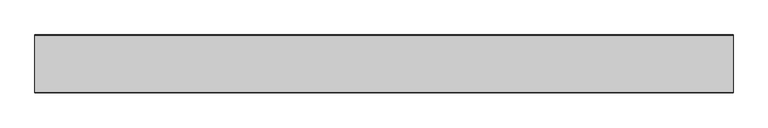
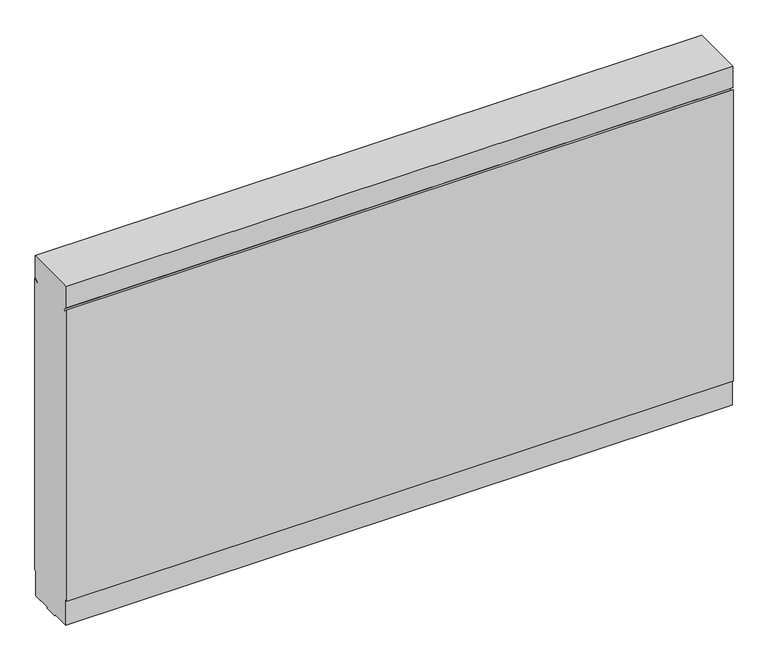
"""IFC4 building model written with IfcOpenShell, lengths in millimetres: proxy geometry, Generic Models 7:Generic Models 1:5:Generic Models 1:5 : Generic Models 7:Generic Models 1:337419:18 : Generic Models 7:Generic Models 1:5:Generic Models 1:5 : Generic Models 7:Generic Models 1:337419:311462."""

from ifc_helpers import new_model, si_unit, frame, origin, place, context, project, spatial, polyline, outline, extrude, source, transform, mapped, element, save


def generic_models_4640aef3(model_context):
    return source(origin(), model_context, "Body", "SweptSolid", [
        extrude(outline(polyline([(-578799.0788841, 103.1875), (-578805.4288841, 103.1875), (-578805.4288841, 7.9375), (-578875.2788841, 7.9375), (-578875.2788841, 1.5875), (-578922.9038841, 1.5875), (-578922.9038841, 7.9375), (-578992.7538841, 7.9375), (-578992.7538841, 103.1875), (-578999.1038841, 103.1875), (-578999.1038841, 1217.1846578), (-578985.9025672, 1206.1074377), (-578982.0759722, 1210.667796), (-578996.3257591, 1222.6247869), (-578996.3257591, 1304.8288409), (-578801.8570091, 1304.8288409), (-578801.8570091, 1222.6247869), (-578816.1067959, 1210.667796), (-578812.2802009, 1206.1074376), (-578799.0788841, 1217.1846577), (-578799.0788841, 103.1875)])), frame((593776.1867239, 0.0, 0.0), z_axis=(1.0, 0.0, 0.0), x_axis=(0.0, 1.0, 0.0)), (0.0, 0.0, 1.0), 2406.65),
    ])


if __name__ == "__main__":
    model = new_model("IFC4")
    model_context = context("Model", 3, world=origin())
    ifc_project = project(units=[si_unit("LENGTHUNIT", "METRE", prefix="MILLI")], contexts=[model_context])
    site = spatial("IfcSite", under=ifc_project)
    building = spatial("IfcBuilding", under=site)
    placement = place(None, origin())
    generic_models_shape = generic_models_4640aef3(model_context)
    element("IfcBuildingElementProxy", 1, Name="Generic Models 7:Generic Models 1:5:Generic Models 1:5 : Generic Models 7:Generic Models 1:337419:18 : Generic Models 7:Generic Models 1:5:Generic Models 1:5 : Generic Models 7:Generic Models 1:337419:311462", ObjectType="Generic Models 7:Generic Models 1:5:Generic Models 1:5 : Generic Models 7:Generic Models 1:337419:18 : Generic Models 7:Generic Models 1:5:Generic Models 1:5 : Generic Models 7:Generic Models 1:337419:311462", at=placement, inside=building, context=model_context, shape_type="MappedRepresentation", body=[
        mapped(generic_models_shape, transform((0.0, 0.0, 0.0), x_axis=(1.0, 0.0, 0.0), y_axis=(0.0, 1.0, 0.0), z_axis=(0.0, 0.0, 1.0))),
    ])
    save(model, "model.ifc")

# Revit data of these elements
# Type "Generic Models 7:Generic Models 1:5:Generic Models 1:5 : Generic Models 7:Generic Models 1:337419:18 : Generic Models 7:Generic Models 1:5:Generic Models 1:5 : Generic Models 7:Generic Models 1:337419:311462"
#   NameOverride = "Generic Models 7:Generic Models 1:5:Generic Models 1:5 : Generic Models 7:Generic Models 1:337419:311462"
#   ObjectTypeOverride = "Generic Models 1:5 : Generic Models 7:Generic Models 1:337419"
#   Reference = "Generic Models 1"
#   Tag = "311462"
# Element 1 (IfcBuildingElementProxy, "Generic Models 7:Generic Models 1:5:Generic Models 1:5 : Generic Models 7:Generic Models 1:337419:18 : Generic Models 7:Generic Models 1:5:Generic Models 1:5 : Generic Models 7:Generic Models 1:337419:311462")
#   Materials on its faces: "SIMPLE SAVER INSULATION WITH LINER - COLOR: BLACK"
# Materials
#   "SIMPLE SAVER INSULATION WITH LINER - COLOR: BLACK": class "Unassigned", colour RGB 158 92 175, transparency 0, Cost = 0
